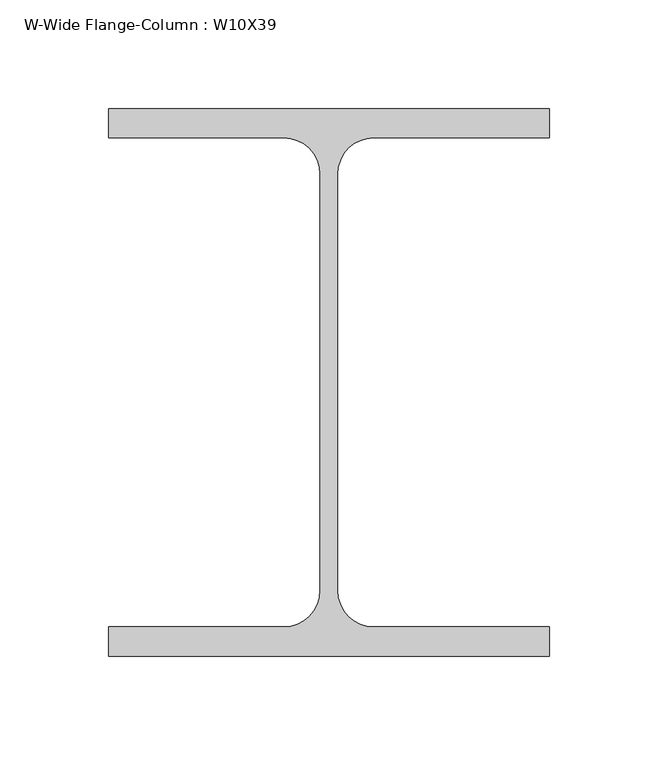
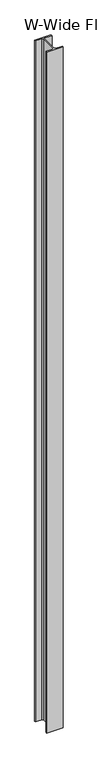
"""IFC4 building model written with IfcOpenShell, lengths in millimetres: column geometry, W-Wide Flange-Column : W10X39."""

from ifc_helpers import new_model, si_unit, point, frame, frame_2d, origin, place, context, project, spatial, polyline, circle_curve, trimmed, segment, composite_curve, outline, extrude, source, transform, mapped, element, save


def w_wide_flange_column_w10x39_67b4d1e6(model_context):
    return source(origin(), model_context, "Body", "SweptSolid", [
        extrude(outline(composite_curve([segment(polyline([(101.473, 125.984), (101.473, 112.522), (20.701, 112.522)]), True, "CONTINUOUS"), segment(trimmed(circle_curve(frame_2d((20.701, 95.8215)), 16.7005), [point((20.701, 112.522))], [point((4.0005, 95.8215))], True, "CARTESIAN"), True, "CONTINUOUS"), segment(polyline([(4.0005, 95.8215), (4.0005, -95.8215)]), True, "CONTINUOUS"), segment(trimmed(circle_curve(frame_2d((20.701, -95.8215)), 16.7005), [point((4.0005, -95.8215))], [point((20.701, -112.522))], True, "CARTESIAN"), True, "CONTINUOUS"), segment(polyline([(20.701, -112.522), (101.473, -112.522), (101.473, -125.984), (-101.473, -125.984), (-101.473, -112.522), (-20.701, -112.522)]), True, "CONTINUOUS"), segment(trimmed(circle_curve(frame_2d((-20.701, -95.8215)), 16.7005), [point((-20.701, -112.522))], [point((-4.0005, -95.8215))], True, "CARTESIAN"), True, "CONTINUOUS"), segment(polyline([(-4.0005, -95.8215), (-4.0005, 95.8215)]), True, "CONTINUOUS"), segment(trimmed(circle_curve(frame_2d((-20.701, 95.8215)), 16.7005), [point((-4.0005, 95.8215))], [point((-20.701, 112.522))], True, "CARTESIAN"), True, "CONTINUOUS"), segment(polyline([(-20.701, 112.522), (-101.473, 112.522), (-101.473, 125.984), (101.473, 125.984)]), True, "CONTINUOUS")], self_intersect=False)), frame((0.0, 0.0, 8756.65), z_axis=(0.0, 0.0, 1.0), x_axis=(1.0, 0.0, 0.0)), (0.0, 0.0, 1.0), 8870.95),
    ])


if __name__ == "__main__":
    model = new_model("IFC4")
    model_context = context("Model", 3, world=origin())
    ifc_project = project(units=[si_unit("LENGTHUNIT", "METRE", prefix="MILLI")], contexts=[model_context])
    site = spatial("IfcSite", under=ifc_project)
    building = spatial("IfcBuilding", under=site)
    placement = place(None, origin())
    w_wide_flange_column_w10x39_shape = w_wide_flange_column_w10x39_67b4d1e6(model_context)
    element("IfcColumn", 1, ObjectType="W-Wide Flange-Column : W10X39", at=placement, inside=building, context=model_context, shape_type="MappedRepresentation", body=[
        mapped(w_wide_flange_column_w10x39_shape, transform((0.0, 0.0, 0.0), x_axis=(1.0, 0.0, 0.0), y_axis=(0.0, 1.0, 0.0), z_axis=(0.0, 0.0, 1.0))),
    ])
    save(model, "model.ifc")

# Revit data of these elements
# Type "W-Wide Flange-Column : W10X39"
#   Assembly Code = "B10"
#   W = 39
#   bf = 0' - 7.99"
#   d = 0' - 9.92"
#   k = 0' - 1 3/16"
#   kr = 0' - 0.6575"
#   tf = 0' - 0.53"
#   tw = 0' - 0.315"
#   A = 0.0798611 SF
#   Structural Material [instance default] = Steel ASTM A992
# Element 1 (IfcColumn, "W-Wide Flange-Column : W10X39")
#   Materials on its faces: "Steel ASTM A992"
# Materials
#   "Steel ASTM A992": class "Metal", colour RGB 199 199 199, transparency 0, Description = "Structural steel 50ksi", Cost = 0
